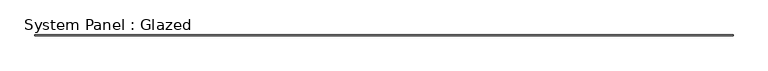
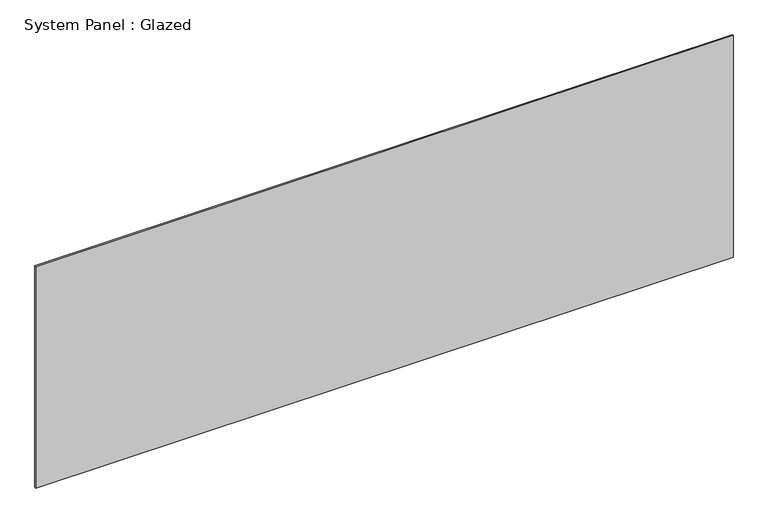
"""IFC4 building model written with IfcOpenShell, lengths in millimetres: plate geometry, System Panel : Glazed."""

from ifc_helpers import new_model, si_unit, origin, origin_with_axes, place, context, project, spatial, polyline, outline, extrude, source, transform, mapped, element, save


def system_panel_glazed_08161773(model_context):
    return source(origin(), model_context, "Body", "SweptSolid", [
        extrude(outline(polyline([(8487.75, 24.5), (-8487.75, 24.5), (-8487.75, 49.5), (8487.75, 49.5), (8487.75, 24.5)])), origin_with_axes(), (0.0, 0.0, 1.0), 5700.0),
    ])


if __name__ == "__main__":
    model = new_model("IFC4")
    model_context = context("Model", 3, world=origin())
    ifc_project = project(units=[si_unit("LENGTHUNIT", "METRE", prefix="MILLI")], contexts=[model_context])
    site = spatial("IfcSite", under=ifc_project)
    building = spatial("IfcBuilding", under=site)
    placement = place(None, origin())
    system_panel_glazed_shape = system_panel_glazed_08161773(model_context)
    element("IfcPlate", 1, ObjectType="System Panel : Glazed", at=placement, inside=building, context=model_context, shape_type="MappedRepresentation", body=[
        mapped(system_panel_glazed_shape, transform((0.0, 0.0, 0.0), x_axis=(1.0, 0.0, 0.0), y_axis=(0.0, 1.0, 0.0), z_axis=(0.0, 0.0, 1.0))),
    ])
    save(model, "model.ifc")

# Revit data of these elements
# Element 1 (IfcPlate, "System Panel : Glazed")
#   Materials on its faces: "Glass"
# Materials
#   "Glass": class "Glass", colour RGB 0 128 192, transparency 0.9
